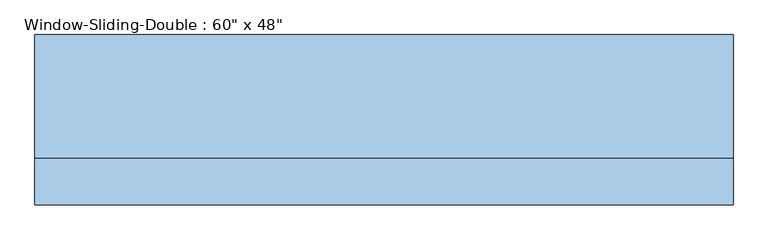
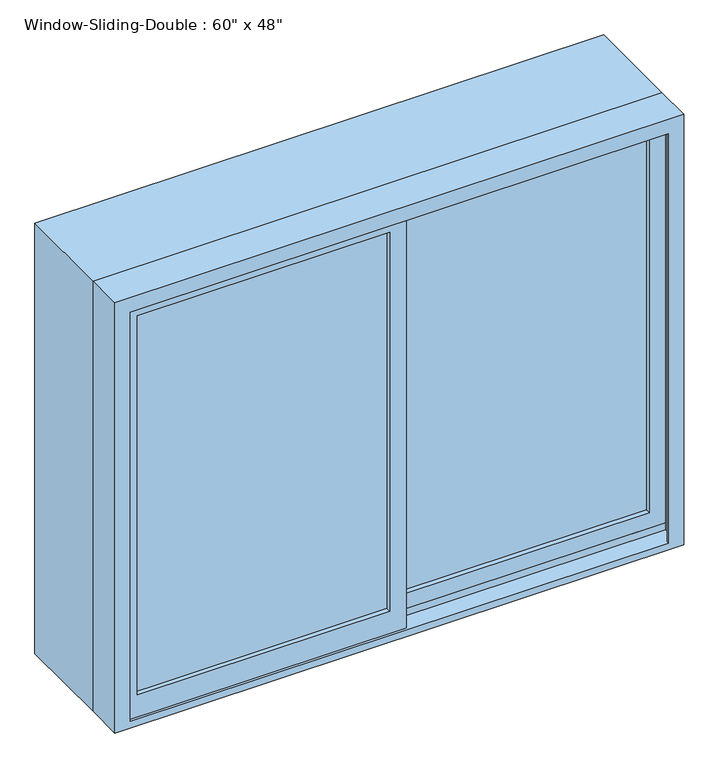
"""IFC4 building model written with IfcOpenShell, lengths in millimetres: window geometry."""

from ifc_helpers import new_model, si_unit, frame, origin, place, context, project, spatial, polyline, outline, extrude, faceted_brep, source, transform, mapped, element, save


def window_a5531389(model_context):
    return source(origin(), model_context, "Body", "SolidModel", [
        faceted_brep([(-762.0, -89.8525, 914.4), (762.0, -89.8525, 914.4), (762.0, -191.4525, 914.4), (-762.0, -191.4525, 914.4), (-721.0778905, -191.4525, 2092.6778905), (-721.0778905, -191.4525, 933.45), (-721.0778905, -185.1025, 933.45), (-721.0778905, -185.1025, 2092.6778905), (-742.95, -185.1025, 933.45), (-742.95, -185.1025, 2114.55), (742.95, -185.1025, 2114.55), (742.95, -185.1025, 933.45), (721.0778905, -185.1025, 933.45), (721.0778905, -185.1025, 2092.6778905), (-742.95, -140.6525, 933.45), (-742.95, -140.6525, 952.5), (-742.95, -96.2025, 952.5), (-742.95, -96.2025, 933.45), (-742.95, -89.8525, 933.45), (-742.95, -89.8525, 2114.55), (-762.0, -89.8525, 2133.6), (762.0, -89.8525, 2133.6), (742.95, -89.8525, 2114.55), (742.95, -89.8525, 933.45), (-762.0, -191.4525, 2133.6), (762.0, -191.4525, 2133.6), (721.0778905, -191.4525, 2092.6778905), (721.0778905, -191.4525, 933.45), (742.95, -96.2025, 933.45), (742.95, -96.2025, 952.5), (742.95, -140.6525, 952.5), (742.95, -140.6525, 933.45)], [[[0, 1, 2, 3]], [[4, 5, 6, 7]], [[7, 6, 8, 9, 10, 11, 12, 13]], [[9, 8, 14, 15, 16, 17, 18, 19]], [[0, 20, 21, 1], [22, 19, 18, 23]], [[24, 20, 0, 3]], [[2, 25, 24, 3], [4, 26, 27, 5]], [[7, 13, 26, 4]], [[9, 19, 22, 10]], [[20, 24, 25, 21]], [[13, 12, 27, 26]], [[22, 23, 28, 29, 30, 31, 11, 10]], [[21, 25, 2, 1]], [[27, 12, 11, 31, 14, 8, 6, 5]], [[31, 30, 15, 14]], [[30, 29, 16, 15]], [[29, 28, 17, 16]], [[18, 17, 28, 23]]]),
        extrude(outline(polyline([(2133.6, 762.0), (2133.6, -762.0), (914.4, -762.0), (914.4, 762.0), (2133.6, 762.0)]), holes=[polyline([(2114.55, -742.95), (2114.55, 742.95), (933.45, 742.95), (933.45, -742.95), (2114.55, -742.95)])]), frame((0.0, -89.8525, 0.0), z_axis=(0.0, 1.0, 0.0), x_axis=(0.0, 0.0, 1.0)), (0.0, 0.0, 1.0), 269.875),
        extrude(outline(polyline([(698.5, -127.9525), (22.225, -127.9525), (22.225, -121.6025), (698.5, -121.6025), (698.5, -127.9525)])), frame((0.0, 0.0, 996.95), z_axis=(0.0, 0.0, 1.0), x_axis=(1.0, 0.0, 0.0)), (0.0, 0.0, 1.0), 1073.15),
        extrude(outline(polyline([(698.5, -115.2525), (22.225, -115.2525), (22.225, -108.9025), (698.5, -108.9025), (698.5, -115.2525)])), frame((0.0, 0.0, 996.95), z_axis=(0.0, 0.0, 1.0), x_axis=(1.0, 0.0, 0.0)), (0.0, 0.0, 1.0), 1073.15),
        extrude(outline(polyline([(-22.225, -172.4025), (-698.5, -172.4025), (-698.5, -166.0525), (-22.225, -166.0525), (-22.225, -172.4025)])), frame((0.0, 0.0, 996.95), z_axis=(0.0, 0.0, 1.0), x_axis=(1.0, 0.0, 0.0)), (0.0, 0.0, 1.0), 1073.15),
        extrude(outline(polyline([(-22.225, -159.7025), (-698.5, -159.7025), (-698.5, -153.3525), (-22.225, -153.3525), (-22.225, -159.7025)])), frame((0.0, 0.0, 996.95), z_axis=(0.0, 0.0, 1.0), x_axis=(1.0, 0.0, 0.0)), (0.0, 0.0, 1.0), 1073.15),
        extrude(outline(polyline([(933.45, 22.225), (2114.55, 22.225), (2114.55, -742.95), (933.45, -742.95), (933.45, 22.225)]), holes=[polyline([(2070.1, -698.5), (2070.1, -22.225), (996.95, -22.225), (996.95, -698.5), (2070.1, -698.5)])]), frame((0.0, -185.1025, 0.0), z_axis=(0.0, 1.0, 0.0), x_axis=(0.0, 0.0, 1.0)), (0.0, 0.0, 1.0), 44.45),
        extrude(outline(polyline([(952.5, -22.225), (952.5, 742.95), (2114.55, 742.95), (2114.55, -22.225), (952.5, -22.225)]), holes=[polyline([(996.95, 698.5), (996.95, 22.225), (2070.1, 22.225), (2070.1, 698.5), (996.95, 698.5)])]), frame((0.0, -140.6525, 0.0), z_axis=(0.0, 1.0, 0.0), x_axis=(0.0, 0.0, 1.0)), (0.0, 0.0, 1.0), 44.45),
    ])


if __name__ == "__main__":
    model = new_model("IFC4")
    model_context = context("Model", 3, world=origin())
    ifc_project = project(units=[si_unit("LENGTHUNIT", "METRE", prefix="MILLI")], contexts=[model_context])
    site = spatial("IfcSite", under=ifc_project)
    building = spatial("IfcBuilding", under=site)
    placement = place(None, origin())
    window_shape = window_a5531389(model_context)
    element("IfcWindow", 1, ObjectType="Window-Sliding-Double : 60\" x 48\"", at=placement, inside=building, context=model_context, shape_type="MappedRepresentation", body=[
        mapped(window_shape, transform((0.0, 0.0, 0.0), x_axis=(1.0, 0.0, 0.0), y_axis=(0.0, 1.0, 0.0), z_axis=(0.0, 0.0, 1.0))),
    ])
    save(model, "model.ifc")

# Revit data of these elements
# Type "Window-Sliding-Double : 60\" x 48\""
#   Type Mark = "13"
#   Fire Rating = "0.5h"
#   Assembly Code = "B2020100"
#   Analytic Construction = "Double glazing - domestic"
#   Window Inset [instance default] = 0' - 0"
#   Wall Thickness [instance default] = 0' - 6"
#   Visual Light Transmittance = 0.81
#   Thermal Resistance (R) = 1.8146 (h·ft²·°F)/BTU
#   Solar Heat Gain Coefficient = 0.76
#   Muntin Width = 2' - 2 5/8"
#   Muntin Height = 3' - 6 1/4"
#   Interior Wall Closure [instance default] = 0' - 2 3/4"
#   Heat Transfer Coefficient (U) = 0.5511 BTU/(h·ft²·°F)
#   Frame Extension [instance default] = 0' - 0 1/4"
#   Exterior Wall Closure [instance default] = 0' - 1 1/4"
#   Rough Width = 5' - 0 1/2"
#   Rough Height = 4' - 0 1/2"
#   Height = 4' - 0"
#   Extension Jamb [instance default] = 0' - 2 3/4"
#   Default Sill Height = 3' - 0"
#   Width = 5' - 0"
#   Interior Trim Visibility [instance default] = yes
#   Indicator Visibility [instance default] = yes
#   Exterior Trim Visibility [instance default] = yes
#   Muntin Visibility = yes
#   Extension Jamb Visibility [instance default] = yes
#   Define Thermal Properties by = 1
#   Muntin Pattern = Muntin Pattern_2x2 : Muntin Pattern_2x2
#   Interior Trim Material = Cherry
#   Interior Trim = Trim-Window-Interior-Flat : Picture Frame
#   Interior Frame Material = Cherry
#   Glass Panel Material = Glass, Clear Glazing
#   Exterior Trim Material = PVC, Flexible
#   Exterior Trim = Trim-Window-Exterior-Flat : with Sill
#   Exterior Frame Material = PVC, Flexible
#   Wall Closure = (empty or 0)
# Element 1 (IfcWindow, "Window-Sliding-Double : 60\" x 48\"")
#   Wall Thickness = 1' - 1 7/8"
#   Extension Jamb = 0' - 10 5/8"
#   Materials on its faces: "Cherry", "Glass, Clear Glazing", "PVC, Flexible"
# Materials
#   "Cherry": class "Wood", colour RGB 157 77 38, transparency 0, Description = "Prunus Serotina", Cost = 0
#   "Glass, Clear Glazing": class "Glass", colour RGB 120 120 120, transparency 0, Description = "Clear glazing", Cost = 0
#   "PVC, Flexible": class "Plastic", colour RGB 178 178 178, transparency 0, Description = "Flexible polyvinyl chloride", Cost = 0
